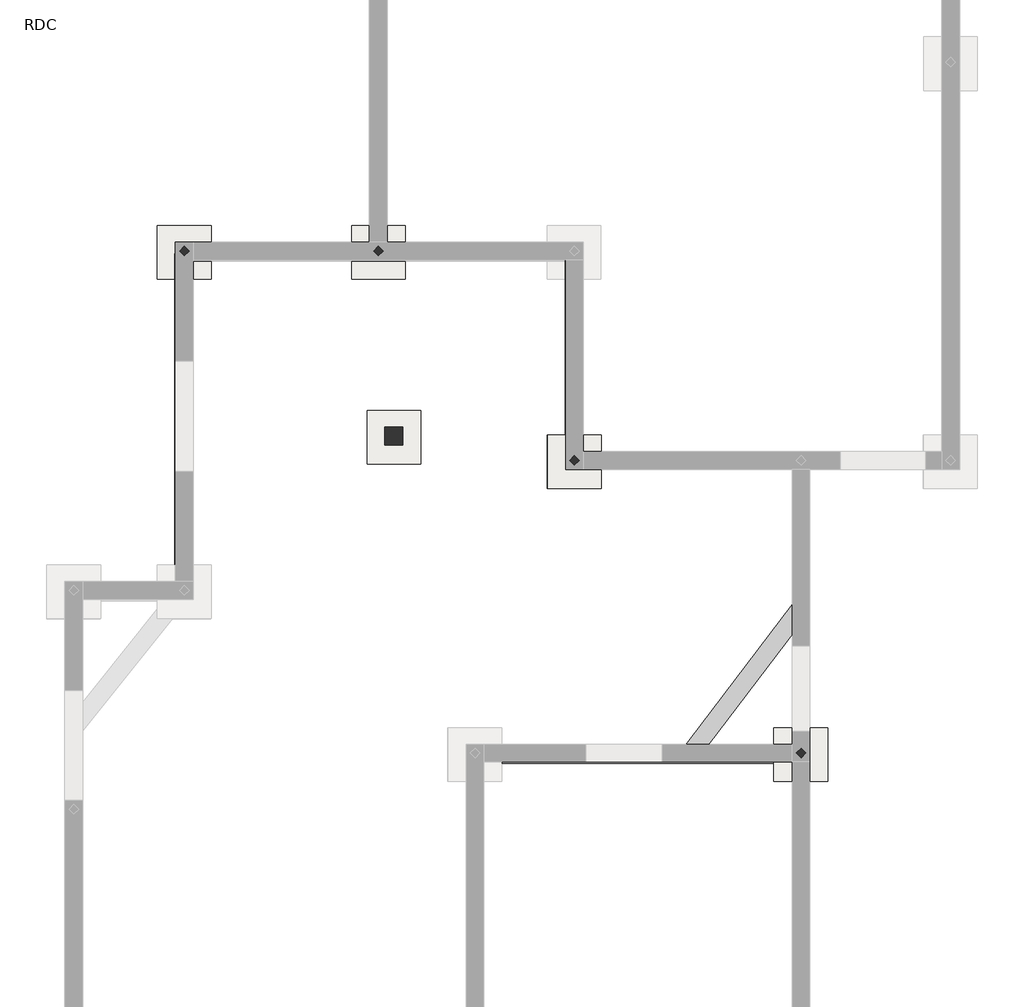
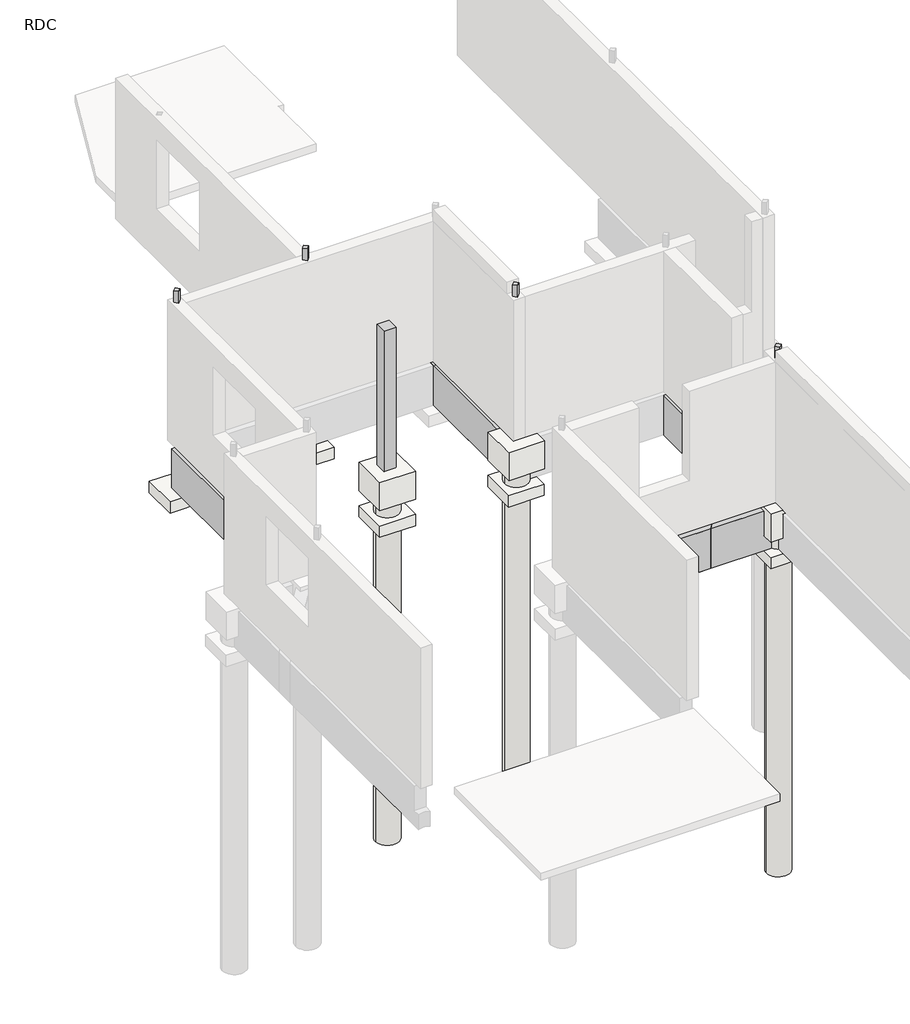
# One storey, part 4 of 5: 11 slabs, 7 beams, 5 columns.
"""IFC4 building model written with IfcOpenShell, lengths in millimetres."""

from ifc_helpers import new_model, si_unit, point, frame, frame_2d, origin, origin_with_axes, place, context, project, spatial, polyline, circle_curve, trimmed, segment, composite_curve, outline, extrude, faceted_brep, element, save
from ifc_brep_helpers import plane_surface, cylinder_surface, revolved_surface, advanced_brep

model = new_model("IFC4")

# Units and contexts
model_context = context("Model", 3, world=origin())
ifc_project = project(units=[si_unit("LENGTHUNIT", "METRE", prefix="MILLI")], contexts=[model_context])

# Site, building, storey
site = spatial("IfcSite", under=ifc_project)
building = spatial("IfcBuilding", under=site)
storey = spatial("IfcBuildingStorey", under=building, Name="RDC", Elevation=0.0)

# Beams
placement = place(None, origin())
element("IfcBeam", 1, ObjectType="Longrine BA : 20x70ht", at=placement, inside=storey, context=model_context, shape_type="AdvancedBrep", body=[
    advanced_brep(
    [(-4817.1649422, 2835.3224776, -67.0), (-4817.1649422, 2835.3224776, -767.0), (-4904.4649416, 2835.3224776, -767.0), (-5017.1649422, 2835.3224776, -767.0), (-5017.1649422, 2835.3224776, -67.0), (-4904.4649416, 2835.3224776, -67.0), (-4817.1649422, 2748.0224782, -67.0), (-4817.1649422, -644.3733983, -67.0), (-4817.1649422, -644.3733983, -500.0), (-4817.1649422, -768.6233971, -500.0), (-4817.1649422, -768.6233971, -767.0), (-4817.1649422, 2748.0224782, -767.0), (-5017.1649422, -773.8722262, -767.0), (-5017.1649422, -773.8722262, -500.0), (-5017.1649422, -644.3733983, -500.0), (-5017.1649422, -644.3733983, -67.0)],
    [
        (0, 1),
        (1, 2),
        (2, 3),
        (3, 4),
        (4, 5),
        (5, 0),
        (0, 6),
        (6, 7),
        (7, 8),
        (8, 9),
        (9, 10),
        (10, 11),
        (11, 1),
        (10, 12, circle_curve(frame((-4912.6214092, -944.3733983, -767.0), z_axis=(0.0, 0.0, 1.0), x_axis=(1.0, 0.0, 0.0)), 200.0)),
        (12, 3),
        (12, 13),
        (13, 14),
        (14, 15),
        (15, 4),
        (15, 7),
        (9, 13, circle_curve(frame((-4912.6214092, -944.3733983, -500.0), z_axis=(0.0, 0.0, 1.0), x_axis=(1.0, 0.0, 0.0)), 200.0)),
        (8, 14),
    ],
    [
        plane_surface(frame((-4817.1649422, 2835.3224776, -67.0), z_axis=(0.0, 1.0, 0.0), x_axis=(0.0, 0.0, -1.0))),
        plane_surface(frame((-4817.1649422, 2835.3224776, -67.0), z_axis=(1.0, 0.0, 0.0), x_axis=(0.0, -1.0, 0.0))),
        plane_surface(frame((-4817.1649422, 2835.3224776, -767.0), z_axis=(0.0, 0.0, -1.0), x_axis=(0.0, -1.0, 0.0))),
        plane_surface(frame((-5017.1649422, 2835.3224776, -767.0), z_axis=(-1.0, 0.0, 0.0), x_axis=(0.0, -1.0, 0.0))),
        plane_surface(frame((-5017.1649422, 2835.3224776, -67.0), z_axis=(0.0, 0.0, 1.0), x_axis=(0.0, -1.0, 0.0))),
        revolved_surface(polyline([(-4712.6214092, -944.3733983, -500.0), (-4712.6214092, -944.3733983, -767.0)]), (-4912.6214092, -944.3733983, -6600.0), (0.0, 0.0, 1.0)),
        plane_surface(frame((-5212.6214092, -644.3733983, -500.0), z_axis=(0.0, 0.0, 1.0), x_axis=(1.0, 0.0, 0.0))),
        plane_surface(frame((-4612.6214092, -644.3733983, 0.0), z_axis=(0.0, -1.0, 0.0), x_axis=(0.0, 0.0, -1.0))),
    ],
    [
        (0, [[1, 2, 3, 4, 5, 6]]),
        (1, [[-1, 7, 8, 9, 10, 11, 12, 13]]),
        (2, [[-3, -2, -13, -12, 14, 15]]),
        (3, [[-4, -15, 16, 17, 18, 19]]),
        (4, [[-6, -5, -19, 20, -8, -7]]),
        (5, [[-14, -11, 21, -16]]),
        (6, [[22, -17, -21, -10]]),
        (7, [[-22, -9, -20, -18]]),
    ],
),
])
element("IfcBeam", 2, ObjectType="Longrine BA : 20x70ht", at=placement, inside=storey, context=model_context, shape_type="AdvancedBrep", body=[
    advanced_brep(
    [(-659.9771125, 2835.3224776, -67.0), (-459.9771125, 2835.3224776, -67.0), (-459.9771125, 2835.3224776, -767.0), (-659.9771125, 2835.3224776, -767.0), (-659.9771125, 678.5236613, -767.0), (-659.9771125, 678.5236613, -500.0), (-659.9771125, 808.0224787, -500.0), (-659.9771125, 808.0224787, -67.0), (-459.9771125, 683.7724706, -767.0), (-459.9771125, 808.0224787, -67.0), (-459.9771125, 808.0224787, -500.0), (-459.9771125, 683.7724706, -500.0)],
    [
        (0, 1),
        (1, 2),
        (2, 3),
        (3, 0),
        (3, 4),
        (4, 5),
        (5, 6),
        (6, 7),
        (7, 0),
        (2, 8),
        (8, 4, circle_curve(frame((-555.4335965, 508.0224787, -767.0), z_axis=(0.0, 0.0, 1.0), x_axis=(1.0, 0.0, 0.0)), 200.0)),
        (1, 9),
        (9, 10),
        (10, 11),
        (11, 8),
        (7, 9),
        (11, 5, circle_curve(frame((-555.4335965, 508.0224787, -500.0), z_axis=(0.0, 0.0, 1.0), x_axis=(1.0, 0.0, 0.0)), 200.0)),
        (10, 6),
    ],
    [
        plane_surface(frame((-659.9771125, 2835.3224776, -67.0), z_axis=(0.0, 1.0, 0.0), x_axis=(0.0, 0.0, 1.0))),
        plane_surface(frame((-659.9771125, 536.535368, -417.0), z_axis=(-1.0, 0.0, 0.0), x_axis=(0.0, 0.0, -1.0))),
        plane_surface(frame((-559.9771125, 536.535368, -767.0), z_axis=(0.0, 0.0, -1.0), x_axis=(1.0, 0.0, 0.0))),
        plane_surface(frame((-459.9771125, 536.535368, -417.0), z_axis=(1.0, 0.0, 0.0), x_axis=(0.0, 0.0, 1.0))),
        plane_surface(frame((-559.9771125, 536.535368, -67.0), z_axis=(0.0, 0.0, 1.0), x_axis=(-1.0, 0.0, 0.0))),
        revolved_surface(polyline([(-355.4335965, 508.0224787, -500.0), (-355.4335965, 508.0224787, -767.0)]), (-555.4335965, 508.0224787, -6600.0), (0.0, 0.0, 1.0)),
        plane_surface(frame((-855.4335965, 808.0224787, -500.0), z_axis=(0.0, 0.0, 1.0), x_axis=(1.0, 0.0, 0.0))),
        plane_surface(frame((-255.4335965, 808.0224787, 0.0), z_axis=(0.0, -1.0, 0.0), x_axis=(0.0, 0.0, -1.0))),
    ],
    [
        (0, [[1, 2, 3, 4]]),
        (1, [[-4, 5, 6, 7, 8, 9]]),
        (2, [[-3, 10, 11, -5]]),
        (3, [[-2, 12, 13, 14, 15, -10]]),
        (4, [[-1, -9, 16, -12]]),
        (5, [[-11, -15, 17, -6]]),
        (6, [[18, -7, -17, -14]]),
        (7, [[-18, -13, -16, -8]]),
    ],
),
])
element("IfcBeam", 3, ObjectType="Longrine BA : 20x70ht", at=placement, inside=storey, context=model_context, shape_type="AdvancedBrep", body=[
    advanced_brep(
    [(1874.5663639, 423.8353673, -67.0), (1874.5663639, 423.8353673, -767.0), (1874.5663639, -2586.2275277, -767.0), (1874.5663639, -2586.2275277, -500.0), (1874.5663639, -2461.9775197, -500.0), (1874.5663639, -2461.9775197, -67.0), (2074.5663639, 423.8353673, -767.0), (2074.5663639, -2591.4763371, -767.0), (2074.5663639, 423.8353673, -67.0), (2074.5663639, -2461.9775197, -67.0), (2074.5663639, -2461.9775197, -500.0), (2074.5663639, -2591.4763371, -500.0)],
    [
        (0, 1),
        (1, 2),
        (2, 3),
        (3, 4),
        (4, 5),
        (5, 0),
        (1, 6),
        (6, 7),
        (7, 2, circle_curve(frame((1970.0228479, -2761.9775197, -767.0), z_axis=(0.0, 0.0, 1.0), x_axis=(1.0, 0.0, 0.0)), 200.0)),
        (6, 8),
        (8, 9),
        (9, 10),
        (10, 11),
        (11, 7),
        (8, 0),
        (5, 9),
        (11, 3, circle_curve(frame((1970.0228479, -2761.9775197, -500.0), z_axis=(0.0, 0.0, 1.0), x_axis=(1.0, 0.0, 0.0)), 200.0)),
        (10, 4),
    ],
    [
        plane_surface(frame((1874.5663639, -2749.277519, -417.0), z_axis=(-1.0, 0.0, 0.0), x_axis=(0.0, 0.0, -1.0))),
        plane_surface(frame((1974.5663639, -2749.277519, -767.0), z_axis=(0.0, 0.0, -1.0), x_axis=(1.0, 0.0, 0.0))),
        plane_surface(frame((2074.5663639, -2749.277519, -417.0), z_axis=(1.0, 0.0, 0.0), x_axis=(0.0, 0.0, 1.0))),
        plane_surface(frame((1974.5663639, -2749.277519, -67.0), z_axis=(0.0, 0.0, 1.0), x_axis=(-1.0, 0.0, 0.0))),
        revolved_surface(polyline([(2170.0228478999998, -2761.9775197, -500.0), (2170.0228478999998, -2761.9775197, -767.0)]), (1970.0228479, -2761.9775197, -6600.0), (0.0, 0.0, 1.0)),
        plane_surface(frame((3631.8663992, 423.8353673, -417.0), z_axis=(0.0, 1.0, 0.0), x_axis=(0.0, 0.0, -1.0))),
        plane_surface(frame((1670.0228479, -2461.9775197, -500.0), z_axis=(0.0, 0.0, 1.0), x_axis=(1.0, 0.0, 0.0))),
        plane_surface(frame((2270.0228479, -2461.9775197, 0.0), z_axis=(0.0, -1.0, 0.0), x_axis=(0.0, 0.0, -1.0))),
    ],
    [
        (0, [[1, 2, 3, 4, 5, 6]]),
        (1, [[7, 8, 9, -2]]),
        (2, [[10, 11, 12, 13, 14, -8]]),
        (3, [[15, -6, 16, -11]]),
        (4, [[-9, -14, 17, -3]]),
        (5, [[-1, -15, -10, -7]]),
        (6, [[18, -4, -17, -13]]),
        (7, [[-18, -12, -16, -5]]),
    ],
),
])
element("IfcBeam", 4, ObjectType="Longrine BA : 20x70ht", at=placement, inside=storey, context=model_context, shape_type="AdvancedBrep", body=[
    advanced_brep(
    [(1796.8177671, -2861.9775197, -767.0), (1796.8177671, -2861.9775197, -500.0), (1670.0228479, -2861.9775197, -500.0), (1670.0228479, -2861.9775197, -67.0), (-1366.4904447, -2861.9775197, -67.0), (-1366.4904447, -2861.9775197, -500.0), (-1491.844941, -2861.9775197, -500.0), (-1491.844941, -2861.9775197, -767.0), (-1466.4904447, -2764.5149728, -767.0), (-1494.7753589, -2661.9775197, -767.0), (1796.8177671, -2661.9775197, -767.0), (1770.0228479, -2761.9775197, -767.0), (1796.8177671, -2661.9775197, -500.0), (-1494.7753589, -2661.9775197, -500.0), (-1366.4904447, -2661.9775197, -500.0), (-1366.4904447, -2661.9775197, -67.0), (1670.0228479, -2661.9775197, -67.0), (1670.0228479, -2661.9775197, -500.0), (-1466.4904447, -2764.5149728, -500.0), (1770.0228479, -2761.9775197, -500.0)],
    [
        (0, 1),
        (1, 2),
        (2, 3),
        (3, 4),
        (4, 5),
        (5, 6),
        (6, 7),
        (7, 0),
        (7, 8, circle_curve(frame((-1666.4904447, -2764.5149728, -767.0), z_axis=(0.0, 0.0, 1.0), x_axis=(1.0, 0.0, 0.0)), 200.0)),
        (8, 9, circle_curve(frame((-1666.4904447, -2764.5149728, -767.0), z_axis=(0.0, 0.0, 1.0), x_axis=(1.0, 0.0, 0.0)), 200.0)),
        (9, 10),
        (10, 11, circle_curve(frame((1970.0228479, -2761.9775197, -767.0), z_axis=(0.0, 0.0, 1.0), x_axis=(1.0, 0.0, 0.0)), 200.0)),
        (11, 0, circle_curve(frame((1970.0228479, -2761.9775197, -767.0), z_axis=(0.0, 0.0, 1.0), x_axis=(1.0, 0.0, 0.0)), 200.0)),
        (12, 10),
        (9, 13),
        (13, 14),
        (14, 15),
        (15, 16),
        (16, 17),
        (17, 12),
        (3, 16),
        (15, 4),
        (6, 18, circle_curve(frame((-1666.4904447, -2764.5149728, -500.0), z_axis=(0.0, 0.0, 1.0), x_axis=(1.0, 0.0, 0.0)), 200.0)),
        (18, 8),
        (18, 13, circle_curve(frame((-1666.4904447, -2764.5149728, -500.0), z_axis=(0.0, 0.0, 1.0), x_axis=(1.0, 0.0, 0.0)), 200.0)),
        (11, 19),
        (19, 1, circle_curve(frame((1970.0228479, -2761.9775197, -500.0), z_axis=(0.0, 0.0, 1.0), x_axis=(1.0, 0.0, 0.0)), 200.0)),
        (12, 19, circle_curve(frame((1970.0228479, -2761.9775197, -500.0), z_axis=(0.0, 0.0, 1.0), x_axis=(1.0, 0.0, 0.0)), 200.0)),
        (17, 2),
        (5, 14),
    ],
    [
        plane_surface(frame((1961.8663633, -2861.9775197, -417.0), z_axis=(0.0, -1.0, 0.0), x_axis=(0.0, 0.0, -1.0))),
        plane_surface(frame((1961.8663633, -2761.9775197, -767.0), z_axis=(0.0, 0.0, -1.0), x_axis=(0.0, 1.0, 0.0))),
        plane_surface(frame((1961.8663633, -2661.9775197, -417.0), z_axis=(0.0, 1.0, 0.0), x_axis=(0.0, 0.0, 1.0))),
        plane_surface(frame((1961.8663633, -2761.9775197, -67.0), z_axis=(0.0, 0.0, 1.0), x_axis=(0.0, -1.0, 0.0))),
        revolved_surface(polyline([(-1466.4904447, -2764.5149728, -500.0), (-1466.4904447, -2764.5149728, -767.0)]), (-1666.4904447, -2764.5149728, -6600.0), (0.0, 0.0, 1.0)),
        revolved_surface(polyline([(2170.0228478999998, -2761.9775197, -500.0), (2170.0228478999998, -2761.9775197, -767.0)]), (1970.0228479, -2761.9775197, -6600.0), (0.0, 0.0, 1.0)),
        plane_surface(frame((1670.0228479, -2461.9775197, -500.0), z_axis=(0.0, 0.0, 1.0), x_axis=(1.0, 0.0, 0.0))),
        plane_surface(frame((1670.0228479, -2461.9775197, 0.0), z_axis=(1.0, 0.0, 0.0), x_axis=(0.0, 0.0, -1.0))),
        plane_surface(frame((-1966.4904447, -2464.5149728, -500.0), z_axis=(0.0, 0.0, 1.0), x_axis=(1.0, 0.0, 0.0))),
        plane_surface(frame((-1366.4904447, -3064.5149728, 0.0), z_axis=(-1.0, 0.0, 0.0), x_axis=(0.0, 0.0, -1.0))),
    ],
    [
        (0, [[1, 2, 3, 4, 5, 6, 7, 8]]),
        (1, [[9, 10, 11, 12, 13, -8]]),
        (2, [[14, -11, 15, 16, 17, 18, 19, 20]]),
        (3, [[21, -18, 22, -4]]),
        (4, [[-9, -7, 23, 24]]),
        (4, [[-10, -24, 25, -15]]),
        (5, [[-1, -13, 26, 27]]),
        (5, [[-26, -12, -14, 28]]),
        (6, [[29, -2, -27, -28, -20]]),
        (7, [[-29, -19, -21, -3]]),
        (8, [[30, -16, -25, -23, -6]]),
        (9, [[-30, -5, -22, -17]]),
    ],
),
])
element("IfcBeam", 5, ObjectType="Longrine BA : 20x70ht", at=placement, inside=storey, context=model_context, shape_type="SweptSolid", body=[
    extrude(outline(polyline([(2074.5663639, -830.5010844), (2074.5663639, -1160.7070139), (779.5785033, -2861.9775197), (528.2294858, -2861.9775197), (2074.5663639, -830.5010844)])), frame((0.0, 0.0, -767.0), z_axis=(0.0, 0.0, 1.0), x_axis=(1.0, 0.0, 0.0)), (0.0, 0.0, 1.0), 700.0),
])
element("IfcBeam", 6, ObjectType="Longrine BA : 20x70ht", at=placement, inside=storey, context=model_context, shape_type="AdvancedBrep", body=[
    advanced_brep(
    [(-459.9771125, 2835.3224776, -67.0), (-459.9771125, 2835.3224776, -767.0), (-572.6771131, 2835.3224776, -767.0), (-572.6771131, 2835.3224776, -67.0), (-459.9771125, 808.0224787, -67.0), (-459.9771125, 808.0224787, -500.0), (-459.9771125, 683.7724706, -500.0), (-459.9771125, 683.7724706, -767.0), (-659.9771125, 678.5236613, -767.0), (-659.9771125, 2748.0224782, -767.0), (-572.6771131, 2748.0224782, -767.0), (-659.9771125, 2748.0224782, -67.0), (-659.9771125, 678.5236613, -500.0), (-659.9771125, 808.0224787, -500.0), (-659.9771125, 808.0224787, -67.0), (-572.6771131, 2748.0224782, -67.0)],
    [
        (0, 1),
        (1, 2),
        (2, 3),
        (3, 0),
        (0, 4),
        (4, 5),
        (5, 6),
        (6, 7),
        (7, 1),
        (7, 8, circle_curve(frame((-555.4335965, 508.0224787, -767.0), z_axis=(0.0, 0.0, 1.0), x_axis=(1.0, 0.0, 0.0)), 200.0)),
        (8, 9),
        (9, 10),
        (10, 2),
        (11, 9),
        (8, 12),
        (12, 13),
        (13, 14),
        (14, 11),
        (3, 15),
        (15, 11),
        (14, 4),
        (15, 10),
        (6, 12, circle_curve(frame((-555.4335965, 508.0224787, -500.0), z_axis=(0.0, 0.0, 1.0), x_axis=(1.0, 0.0, 0.0)), 200.0)),
        (5, 13),
    ],
    [
        plane_surface(frame((-459.9771125, 2835.3224776, -67.0), z_axis=(0.0, 1.0, 0.0), x_axis=(0.0, 0.0, -1.0))),
        plane_surface(frame((-459.9771125, 2835.3224776, -417.0), z_axis=(1.0, 0.0, 0.0), x_axis=(0.0, 0.0, -1.0))),
        plane_surface(frame((-559.9771125, 2835.3224776, -767.0), z_axis=(0.0, 0.0, -1.0), x_axis=(-1.0, 0.0, 0.0))),
        plane_surface(frame((-659.9771125, 2835.3224776, -417.0), z_axis=(-1.0, 0.0, 0.0), x_axis=(0.0, 0.0, 1.0))),
        plane_surface(frame((-559.9771125, 2835.3224776, -67.0), z_axis=(0.0, 0.0, 1.0), x_axis=(1.0, 0.0, 0.0))),
        plane_surface(frame((-4904.4649416, 2748.0224782, -417.0), z_axis=(0.0, 1.0, 0.0), x_axis=(0.0, 0.0, 1.0))),
        revolved_surface(polyline([(-355.4335965, 508.0224787, -500.0), (-355.4335965, 508.0224787, -767.0)]), (-555.4335965, 508.0224787, -6600.0), (0.0, 0.0, 1.0)),
        plane_surface(frame((-572.6771131, 2948.0224782, -67.0), z_axis=(-1.0, 0.0, 0.0), x_axis=(0.0, 0.0, 1.0))),
        plane_surface(frame((-855.4335965, 808.0224787, -500.0), z_axis=(0.0, 0.0, 1.0), x_axis=(1.0, 0.0, 0.0))),
        plane_surface(frame((-255.4335965, 808.0224787, 0.0), z_axis=(0.0, -1.0, 0.0), x_axis=(0.0, 0.0, -1.0))),
    ],
    [
        (0, [[1, 2, 3, 4]]),
        (1, [[-1, 5, 6, 7, 8, 9]]),
        (2, [[-2, -9, 10, 11, 12, 13]]),
        (3, [[14, -11, 15, 16, 17, 18]]),
        (4, [[-4, 19, 20, -18, 21, -5]]),
        (5, [[22, -12, -14, -20]]),
        (6, [[-10, -8, 23, -15]]),
        (7, [[-22, -19, -3, -13]]),
        (8, [[24, -16, -23, -7]]),
        (9, [[-24, -6, -21, -17]]),
    ],
),
])
element("IfcBeam", 7, ObjectType="Longrine BA : 20x70ht", at=placement, inside=storey, context=model_context, shape_type="AdvancedBrep", body=[
    advanced_brep(
    [(678.0743146, -2861.9775197, -767.0), (1796.8177671, -2861.9775197, -767.0), (1796.8177671, -2861.9775197, -500.0), (1670.0228479, -2861.9775197, -500.0), (1670.0228479, -2861.9775197, -67.0), (678.0743146, -2861.9775197, -67.0), (678.0743146, -2665.1211664, -767.0), (680.4672229, -2661.9775197, -767.0), (1796.8177671, -2661.9775197, -767.0), (1770.0228479, -2761.9775197, -767.0), (680.4672229, -2661.9775197, -67.0), (1670.0228479, -2661.9775197, -67.0), (1670.0228479, -2661.9775197, -500.0), (1796.8177671, -2661.9775197, -500.0), (678.0743146, -2665.1211664, -67.0), (1770.0228479, -2761.9775197, -500.0)],
    [
        (0, 1),
        (1, 2),
        (2, 3),
        (3, 4),
        (4, 5),
        (5, 0),
        (0, 6),
        (6, 7),
        (7, 8),
        (8, 9, circle_curve(frame((1970.0228479, -2761.9775197, -767.0), z_axis=(0.0, 0.0, 1.0), x_axis=(1.0, 0.0, 0.0)), 200.0)),
        (9, 1, circle_curve(frame((1970.0228479, -2761.9775197, -767.0), z_axis=(0.0, 0.0, 1.0), x_axis=(1.0, 0.0, 0.0)), 200.0)),
        (7, 10),
        (10, 11),
        (11, 12),
        (12, 13),
        (13, 8),
        (14, 5),
        (4, 11),
        (10, 14),
        (9, 15),
        (15, 2, circle_curve(frame((1970.0228479, -2761.9775197, -500.0), z_axis=(0.0, 0.0, 1.0), x_axis=(1.0, 0.0, 0.0)), 200.0)),
        (13, 15, circle_curve(frame((1970.0228479, -2761.9775197, -500.0), z_axis=(0.0, 0.0, 1.0), x_axis=(1.0, 0.0, 0.0)), 200.0)),
        (12, 3),
        (14, 6),
    ],
    [
        plane_surface(frame((1961.8663633, -2861.9775197, -67.0), z_axis=(0.0, -1.0, 0.0), x_axis=(-1.0, 0.0, 0.0))),
        plane_surface(frame((1961.8663633, -2861.9775197, -767.0), z_axis=(0.0, 0.0, -1.0), x_axis=(-1.0, 0.0, 0.0))),
        plane_surface(frame((1961.8663633, -2661.9775197, -767.0), z_axis=(0.0, 1.0, 0.0), x_axis=(-1.0, 0.0, 0.0))),
        plane_surface(frame((1961.8663633, -2661.9775197, -67.0), z_axis=(0.0, 0.0, 1.0), x_axis=(-1.0, 0.0, 0.0))),
        revolved_surface(polyline([(2170.0228478999998, -2761.9775197, -500.0), (2170.0228478999998, -2761.9775197, -767.0)]), (1970.0228479, -2761.9775197, -6600.0), (0.0, 0.0, 1.0)),
        plane_surface(frame((1670.0228479, -2461.9775197, -500.0), z_axis=(0.0, 0.0, 1.0), x_axis=(1.0, 0.0, 0.0))),
        plane_surface(frame((1670.0228479, -2461.9775197, 0.0), z_axis=(1.0, 0.0, 0.0), x_axis=(0.0, 0.0, -1.0))),
        plane_surface(frame((678.0743146, -2761.9775197, -417.0), z_axis=(-1.0, 0.0, 0.0), x_axis=(0.0, -1.0, 0.0))),
        plane_surface(frame((571.6677663, -2804.9111426, -67.0), z_axis=(-0.7957063128923657, 0.605682642663001, 0.0), x_axis=(0.605682642663001, 0.7957063128923657, 0.0))),
    ],
    [
        (0, [[1, 2, 3, 4, 5, 6]]),
        (1, [[-1, 7, 8, 9, 10, 11]]),
        (2, [[12, 13, 14, 15, 16, -9]]),
        (3, [[17, -5, 18, -13, 19]]),
        (4, [[-11, 20, 21, -2]]),
        (4, [[-10, -16, 22, -20]]),
        (5, [[23, -3, -21, -22, -15]]),
        (6, [[-23, -14, -18, -4]]),
        (7, [[-6, -17, 24, -7]]),
        (8, [[-8, -24, -19, -12]]),
    ],
),
])

# Columns
element("IfcColumn", 8, ObjectType="CV : CV", at=placement, inside=storey, context=model_context, shape_type="Brep", body=[
    faceted_brep([(-4912.6214092, 2916.8683755, 2710.0), (-4965.6544178, 2863.8353669, 2710.0), (-4912.6214092, 2810.8023583, 2710.0), (-4859.5884006, 2863.8353669, 2710.0), (-4912.6214092, 2916.8683755, 0.0), (-4859.5884006, 2863.8353669, 0.0), (-4912.6214092, 2810.8023583, 0.0), (-4965.6544178, 2863.8353669, 0.0), (-4912.6214092, 2916.8683755, 2500.0), (-4965.6544178, 2863.8353669, 2500.0), (-4912.6214092, 2810.8023583, 2500.0), (-4859.5884006, 2863.8353669, 2500.0)], [[[0, 1, 2, 3]], [[4, 5, 6, 7]], [[1, 0, 8, 4, 7, 9]], [[2, 1, 9, 7, 6, 10]], [[3, 2, 10, 6, 5, 11]], [[0, 3, 11, 5, 4, 8]]]),
    faceted_brep([(-4859.5884006, 2863.8353669, 2710.0), (-4912.6214092, 2916.8683755, 2710.0), (-4965.6544178, 2863.8353669, 2710.0), (-4912.6214092, 2810.8023583, 2710.0), (-4859.5884006, 2863.8353669, 0.0), (-4912.6214092, 2810.8023583, 0.0), (-4965.6544178, 2863.8353669, 0.0), (-4912.6214092, 2916.8683755, 0.0), (-4859.5884006, 2863.8353669, 2500.0), (-4912.6214092, 2916.8683755, 2500.0), (-4965.6544178, 2863.8353669, 2500.0), (-4912.6214092, 2810.8023583, 2500.0)], [[[0, 1, 2, 3]], [[4, 5, 6, 7]], [[1, 0, 8, 4, 7, 9]], [[2, 1, 9, 7, 6, 10]], [[3, 2, 10, 6, 5, 11]], [[0, 3, 11, 5, 4, 8]]]),
])
element("IfcColumn", 9, ObjectType="CV : CV", at=placement, inside=storey, context=model_context, shape_type="Brep", body=[
    faceted_brep([(-2745.4336004, 2916.8683755, 2710.0), (-2798.466609, 2863.8353669, 2710.0), (-2745.4336004, 2810.8023583, 2710.0), (-2692.4005918, 2863.8353669, 2710.0), (-2745.4336004, 2916.8683755, 0.0), (-2692.4005918, 2863.8353669, 0.0), (-2745.4336004, 2810.8023583, 0.0), (-2798.466609, 2863.8353669, 0.0), (-2745.4336004, 2916.8683755, 2500.0), (-2798.466609, 2863.8353669, 2500.0), (-2745.4336004, 2810.8023583, 2500.0), (-2692.4005918, 2863.8353669, 2500.0)], [[[0, 1, 2, 3]], [[4, 5, 6, 7]], [[1, 0, 8, 4, 7, 9]], [[2, 1, 9, 7, 6, 10]], [[3, 2, 10, 6, 5, 11]], [[0, 3, 11, 5, 4, 8]]]),
    faceted_brep([(-2692.4005918, 2863.8353669, 2710.0), (-2745.4336004, 2916.8683755, 2710.0), (-2798.466609, 2863.8353669, 2710.0), (-2745.4336004, 2810.8023583, 2710.0), (-2692.4005918, 2863.8353669, 0.0), (-2745.4336004, 2810.8023583, 0.0), (-2798.466609, 2863.8353669, 0.0), (-2745.4336004, 2916.8683755, 0.0), (-2692.4005918, 2863.8353669, 2500.0), (-2745.4336004, 2916.8683755, 2500.0), (-2798.466609, 2863.8353669, 2500.0), (-2745.4336004, 2810.8023583, 2500.0)], [[[0, 1, 2, 3]], [[4, 5, 6, 7]], [[1, 0, 8, 4, 7, 9]], [[2, 1, 9, 7, 6, 10]], [[3, 2, 10, 6, 5, 11]], [[0, 3, 11, 5, 4, 8]]]),
])
element("IfcColumn", 10, ObjectType="CV : CV", at=placement, inside=storey, context=model_context, shape_type="Brep", body=[
    faceted_brep([(-555.4335965, 576.8683759, 2710.0), (-608.4666051, 523.8353673, 2710.0), (-555.4335965, 470.8023588, 2710.0), (-502.4005879, 523.8353673, 2710.0), (-555.4335965, 576.8683759, 0.0), (-502.4005879, 523.8353673, 0.0), (-555.4335965, 470.8023588, 0.0), (-608.4666051, 523.8353673, 0.0), (-555.4335965, 576.8683759, 2500.0), (-608.4666051, 523.8353673, 2500.0), (-555.4335965, 470.8023588, 2500.0), (-502.4005879, 523.8353673, 2500.0)], [[[0, 1, 2, 3]], [[4, 5, 6, 7]], [[1, 0, 8, 4, 7, 9]], [[2, 1, 9, 7, 6, 10]], [[3, 2, 10, 6, 5, 11]], [[0, 3, 11, 5, 4, 8]]]),
    faceted_brep([(-502.4005879, 523.8353673, 2710.0), (-555.4335965, 576.8683759, 2710.0), (-608.4666051, 523.8353673, 2710.0), (-555.4335965, 470.8023588, 2710.0), (-502.4005879, 523.8353673, 0.0), (-555.4335965, 470.8023588, 0.0), (-608.4666051, 523.8353673, 0.0), (-555.4335965, 576.8683759, 0.0), (-502.4005879, 523.8353673, 2500.0), (-555.4335965, 576.8683759, 2500.0), (-608.4666051, 523.8353673, 2500.0), (-555.4335965, 470.8023588, 2500.0)], [[[0, 1, 2, 3]], [[4, 5, 6, 7]], [[1, 0, 8, 4, 7, 9]], [[2, 1, 9, 7, 6, 10]], [[3, 2, 10, 6, 5, 11]], [[0, 3, 11, 5, 4, 8]]]),
])
element("IfcColumn", 11, ObjectType="CV : CV", at=placement, inside=storey, context=model_context, shape_type="Brep", body=[
    faceted_brep([(1974.5663639, -2693.1316224, 2710.0), (1921.5333553, -2746.164631, 2710.0), (1974.5663639, -2799.1976396, 2710.0), (2027.5993725, -2746.164631, 2710.0), (1974.5663639, -2693.1316224, 0.0), (2027.5993725, -2746.164631, 0.0), (1974.5663639, -2799.1976396, 0.0), (1921.5333553, -2746.164631, 0.0), (1974.5663639, -2693.1316224, 2500.0), (1921.5333553, -2746.164631, 2500.0), (1974.5663639, -2799.1976396, 2500.0), (2027.5993725, -2746.164631, 2500.0)], [[[0, 1, 2, 3]], [[4, 5, 6, 7]], [[1, 0, 8, 4, 7, 9]], [[2, 1, 9, 7, 6, 10]], [[3, 2, 10, 6, 5, 11]], [[0, 3, 11, 5, 4, 8]]]),
    faceted_brep([(2027.5993725, -2746.164631, 2710.0), (1974.5663639, -2693.1316224, 2710.0), (1921.5333553, -2746.164631, 2710.0), (1974.5663639, -2799.1976396, 2710.0), (2027.5993725, -2746.164631, 0.0), (1974.5663639, -2799.1976396, 0.0), (1921.5333553, -2746.164631, 0.0), (1974.5663639, -2693.1316224, 0.0), (2027.5993725, -2746.164631, 2500.0), (1974.5663639, -2693.1316224, 2500.0), (1921.5333553, -2746.164631, 2500.0), (1974.5663639, -2799.1976396, 2500.0)], [[[0, 1, 2, 3]], [[4, 5, 6, 7]], [[1, 0, 8, 4, 7, 9]], [[2, 1, 9, 7, 6, 10]], [[3, 2, 10, 6, 5, 11]], [[0, 3, 11, 5, 4, 8]]]),
])
element("IfcColumn", 12, ObjectType="Poteau BA : 20x20", at=placement, inside=storey, context=model_context, shape_type="SweptSolid", body=[
    extrude(outline(polyline([(-2475.4327864, 897.5075352), (-2475.4327864, 697.5075352), (-2675.4327864, 697.5075352), (-2675.4327864, 897.5075352), (-2475.4327864, 897.5075352)])), origin_with_axes(), (0.0, 0.0, 1.0), 2500.0),
])

# Slabs
element("IfcSlab", 13, ObjectType="Pieu-Conduite en acier : Diamètre de 400 mm", at=placement, inside=storey, context=model_context, shape_type="SweptSolid", body=[
    extrude(outline(composite_curve([segment(trimmed(circle_curve(frame_2d((-2571.8171747, 781.6946465)), 200.0), [point((-2771.8171747, 781.6946465))], [point((-2371.8171747, 781.6946465))], False, "CARTESIAN"), True, "CONTINUOUS"), segment(trimmed(circle_curve(frame_2d((-2571.8171747, 781.6946465)), 200.0), [point((-2371.8171747, 781.6946465))], [point((-2771.8171747, 781.6946465))], False, "CARTESIAN"), True, "CONTINUOUS")], self_intersect=False)), frame((0.0, 0.0, -6600.0), z_axis=(0.0, 0.0, 1.0), x_axis=(1.0, 0.0, 0.0)), (0.0, 0.0, 1.0), 5630.0),
    extrude(outline(composite_curve([segment(trimmed(circle_curve(frame_2d((-2571.8171747, 781.6946465)), 200.0), [point((-2371.8171747, 781.6946465))], [point((-2771.8171747, 781.6946465))], False, "CARTESIAN"), True, "CONTINUOUS"), segment(trimmed(circle_curve(frame_2d((-2571.8171747, 781.6946465)), 200.0), [point((-2771.8171747, 781.6946465))], [point((-2371.8171747, 781.6946465))], False, "CARTESIAN"), True, "CONTINUOUS")], self_intersect=False)), frame((0.0, 0.0, -770.0), z_axis=(0.0, 0.0, 1.0), x_axis=(1.0, 0.0, 0.0)), (0.0, 0.0, 1.0), 270.0),
])
element("IfcSlab", 14, ObjectType="Pieu-Conduite en acier : Diamètre de 400 mm", at=placement, inside=storey, context=model_context, shape_type="AdvancedBrep", body=[
    advanced_brep(
    [(-755.4335965, 508.0224787, -6600.0), (-355.4335965, 508.0224787, -6600.0), (-755.4335965, 508.0224787, -970.0), (-355.4335965, 508.0224787, -970.0)],
    [
        (0, 1, circle_curve(frame((-555.4335965, 508.0224787, -6600.0), z_axis=(0.0, 0.0, -1.0), x_axis=(1.0, 0.0, 0.0)), 200.0)),
        (1, 0, circle_curve(frame((-555.4335965, 508.0224787, -6600.0), z_axis=(0.0, 0.0, -1.0), x_axis=(1.0, 0.0, 0.0)), 200.0)),
        (2, 3, circle_curve(frame((-555.4335965, 508.0224787, -970.0), z_axis=(0.0, 0.0, 1.0), x_axis=(1.0, 0.0, 0.0)), 200.0)),
        (3, 2, circle_curve(frame((-555.4335965, 508.0224787, -970.0), z_axis=(0.0, 0.0, 1.0), x_axis=(1.0, 0.0, 0.0)), 200.0)),
        (1, 3),
        (2, 0),
    ],
    [
        plane_surface(frame((-355.4335965, 508.0224787, -6600.0), z_axis=(0.0, 0.0, -1.0), x_axis=(0.0, -1.0, 0.0))),
        plane_surface(frame((-859.9771445, 808.0224787, -970.0), z_axis=(0.0, 0.0, 1.0), x_axis=(1.0, 0.0, 0.0))),
        cylinder_surface(frame((-555.4335965, 508.0224787, -6600.0), z_axis=(0.0, 0.0, 1.0), x_axis=(1.0, 0.0, 0.0)), 200.0),
    ],
    [
        (0, [[1, 2]]),
        (1, [[3, 4]]),
        (2, [[-2, 5, -3, 6]]),
        (2, [[-1, -6, -4, -5]]),
    ],
),
    advanced_brep(
    [(-755.4335965, 508.0224787, -770.0), (-355.4335965, 508.0224787, -770.0), (-355.4335965, 508.0224787, -500.0), (-374.0154875, 423.8353673, -500.0), (-755.4335965, 508.0224787, -500.0), (-659.9771125, 678.5236613, -500.0), (-459.9771125, 683.7724706, -500.0), (-392.3878332, 623.850278, -500.0)],
    [
        (0, 1, circle_curve(frame((-555.4335965, 508.0224787, -770.0), z_axis=(0.0, 0.0, 1.0), x_axis=(1.0, 0.0, 0.0)), 200.0)),
        (1, 2),
        (2, 3, circle_curve(frame((-555.4335965, 508.0224787, -500.0), z_axis=(0.0, 0.0, -1.0), x_axis=(1.0, 0.0, 0.0)), 200.0)),
        (3, 4, circle_curve(frame((-555.4335965, 508.0224787, -500.0), z_axis=(0.0, 0.0, -1.0), x_axis=(1.0, 0.0, 0.0)), 200.0)),
        (4, 0),
        (1, 0, circle_curve(frame((-555.4335965, 508.0224787, -770.0), z_axis=(0.0, 0.0, 1.0), x_axis=(1.0, 0.0, 0.0)), 200.0)),
        (4, 5, circle_curve(frame((-555.4335965, 508.0224787, -500.0), z_axis=(0.0, 0.0, -1.0), x_axis=(1.0, 0.0, 0.0)), 200.0)),
        (5, 6, circle_curve(frame((-555.4335965, 508.0224787, -500.0), z_axis=(0.0, 0.0, -1.0), x_axis=(1.0, 0.0, 0.0)), 200.0)),
        (6, 7, circle_curve(frame((-555.4335965, 508.0224787, -500.0), z_axis=(0.0, 0.0, -1.0), x_axis=(1.0, 0.0, 0.0)), 200.0)),
        (7, 2, circle_curve(frame((-555.4335965, 508.0224787, -500.0), z_axis=(0.0, 0.0, -1.0), x_axis=(1.0, 0.0, 0.0)), 200.0)),
    ],
    [
        cylinder_surface(frame((-555.4335965, 508.0224787, -6600.0), z_axis=(0.0, 0.0, 1.0), x_axis=(1.0, 0.0, 0.0)), 200.0),
        plane_surface(frame((-859.9771445, 808.0224787, -770.0), z_axis=(0.0, 0.0, -1.0), x_axis=(-1.0, 0.0, 0.0))),
        plane_surface(frame((-855.4335965, 808.0224787, -500.0), z_axis=(0.0, 0.0, 1.0), x_axis=(1.0, 0.0, 0.0))),
    ],
    [
        (0, [[1, 2, 3, 4, 5]]),
        (0, [[6, -5, 7, 8, 9, 10, -2]]),
        (1, [[-1, -6]]),
        (2, [[-4, -3, -10, -9, -8, -7]]),
    ],
),
])
element("IfcSlab", 15, ObjectType="Pieu-Conduite en acier : Diamètre de 400 mm", at=placement, inside=storey, context=model_context, shape_type="AdvancedBrep", body=[
    advanced_brep(
    [(1770.0228479, -2761.9775197, -6600.0), (2170.0228479, -2761.9775197, -6600.0), (1770.0228479, -2761.9775197, -970.0), (2170.0228479, -2761.9775197, -970.0)],
    [
        (0, 1, circle_curve(frame((1970.0228479, -2761.9775197, -6600.0), z_axis=(0.0, 0.0, -1.0), x_axis=(1.0, 0.0, 0.0)), 200.0)),
        (1, 0, circle_curve(frame((1970.0228479, -2761.9775197, -6600.0), z_axis=(0.0, 0.0, -1.0), x_axis=(1.0, 0.0, 0.0)), 200.0)),
        (2, 3, circle_curve(frame((1970.0228479, -2761.9775197, -970.0), z_axis=(0.0, 0.0, 1.0), x_axis=(1.0, 0.0, 0.0)), 200.0)),
        (3, 2, circle_curve(frame((1970.0228479, -2761.9775197, -970.0), z_axis=(0.0, 0.0, 1.0), x_axis=(1.0, 0.0, 0.0)), 200.0)),
        (1, 3),
        (2, 0),
    ],
    [
        plane_surface(frame((2170.0228479, -2761.9775197, -6600.0), z_axis=(0.0, 0.0, -1.0), x_axis=(0.0, -1.0, 0.0))),
        plane_surface(frame((1670.0228479, -2461.9775197, -970.0), z_axis=(0.0, 0.0, 1.0), x_axis=(1.0, 0.0, 0.0))),
        cylinder_surface(frame((1970.0228479, -2761.9775197, -6600.0), z_axis=(0.0, 0.0, 1.0), x_axis=(1.0, 0.0, 0.0)), 200.0),
    ],
    [
        (0, [[1, 2]]),
        (1, [[3, 4]]),
        (2, [[-2, 5, -3, 6]]),
        (2, [[-1, -6, -4, -5]]),
    ],
),
    advanced_brep(
    [(1770.0228479, -2761.9775197, -770.0), (2170.0228479, -2761.9775197, -770.0), (2170.0228479, -2761.9775197, -500.0), (2074.5557716, -2932.4851965, -500.0), (1874.5489367, -2937.7180451, -500.0), (1796.8177671, -2861.9775197, -500.0), (1770.0228479, -2761.9775197, -500.0), (1796.8281566, -2661.9595268, -500.0), (1874.5663639, -2586.2275277, -500.0), (2074.5663639, -2591.4763371, -500.0)],
    [
        (0, 1, circle_curve(frame((1970.0228479, -2761.9775197, -770.0), z_axis=(0.0, 0.0, 1.0), x_axis=(1.0, 0.0, 0.0)), 200.0)),
        (1, 2),
        (2, 3, circle_curve(frame((1970.0228479, -2761.9775197, -500.0), z_axis=(0.0, 0.0, -1.0), x_axis=(1.0, 0.0, 0.0)), 200.0)),
        (3, 4, circle_curve(frame((1970.0228479, -2761.9775197, -500.0), z_axis=(0.0, 0.0, -1.0), x_axis=(1.0, 0.0, 0.0)), 200.0)),
        (4, 5, circle_curve(frame((1970.0228479, -2761.9775197, -500.0), z_axis=(0.0, 0.0, -1.0), x_axis=(1.0, 0.0, 0.0)), 200.0)),
        (5, 6, circle_curve(frame((1970.0228479, -2761.9775197, -500.0), z_axis=(0.0, 0.0, -1.0), x_axis=(1.0, 0.0, 0.0)), 200.0)),
        (6, 0),
        (1, 0, circle_curve(frame((1970.0228479, -2761.9775197, -770.0), z_axis=(0.0, 0.0, 1.0), x_axis=(1.0, 0.0, 0.0)), 200.0)),
        (6, 7, circle_curve(frame((1970.0228479, -2761.9775197, -500.0), z_axis=(0.0, 0.0, -1.0), x_axis=(1.0, 0.0, 0.0)), 200.0)),
        (7, 8, circle_curve(frame((1970.0228479, -2761.9775197, -500.0), z_axis=(0.0, 0.0, -1.0), x_axis=(1.0, 0.0, 0.0)), 200.0)),
        (8, 9, circle_curve(frame((1970.0228479, -2761.9775197, -500.0), z_axis=(0.0, 0.0, -1.0), x_axis=(1.0, 0.0, 0.0)), 200.0)),
        (9, 2, circle_curve(frame((1970.0228479, -2761.9775197, -500.0), z_axis=(0.0, 0.0, -1.0), x_axis=(1.0, 0.0, 0.0)), 200.0)),
    ],
    [
        cylinder_surface(frame((1970.0228479, -2761.9775197, -6600.0), z_axis=(0.0, 0.0, 1.0), x_axis=(1.0, 0.0, 0.0)), 200.0),
        plane_surface(frame((1670.0228479, -2461.9775197, -770.0), z_axis=(0.0, 0.0, -1.0), x_axis=(-1.0, 0.0, 0.0))),
        plane_surface(frame((1670.0228479, -2461.9775197, -500.0), z_axis=(0.0, 0.0, 1.0), x_axis=(1.0, 0.0, 0.0))),
    ],
    [
        (0, [[1, 2, 3, 4, 5, 6, 7]]),
        (0, [[8, -7, 9, 10, 11, 12, -2]]),
        (1, [[-1, -8]]),
        (2, [[-6, -5, -4, -3, -12, -11, -10, -9]]),
    ],
),
])
element("IfcSlab", 16, ObjectType="Tête de pieux-1 poteau : 60x60x50", at=placement, inside=storey, context=model_context, shape_type="SweptSolid", body=[
    extrude(outline(polyline([(-2271.8171747, 1081.6946465), (-2271.8171747, 481.6946465), (-2871.8171747, 481.6946465), (-2871.8171747, 1081.6946465), (-2271.8171747, 1081.6946465)])), frame((0.0, 0.0, -500.0), z_axis=(0.0, 0.0, 1.0), x_axis=(1.0, 0.0, 0.0)), (0.0, 0.0, 1.0), 500.0),
])
element("IfcSlab", 17, ObjectType="Tête de pieux-1 poteau : 60x60x50", at=placement, inside=storey, context=model_context, shape_type="Brep", body=[
    faceted_brep([(-255.4335965, 808.0224787, 0.0), (-855.4335965, 808.0224787, 0.0), (-855.4335965, 208.0224787, 0.0), (-255.4335965, 208.0224787, 0.0), (-255.4335965, 808.0224787, -500.0), (-255.4335965, 623.8353673, -500.0), (-255.4335965, 423.8353673, -500.0), (-255.4335965, 208.0224787, -500.0), (-855.4335965, 208.0224787, -500.0), (-855.4335965, 808.0224787, -500.0), (-659.9771125, 808.0224787, -500.0), (-459.9771125, 808.0224787, -500.0)], [[[0, 1, 2, 3]], [[4, 5, 6, 7, 8, 9, 10, 11]], [[1, 0, 4, 11, 10, 9]], [[2, 1, 9, 8]], [[3, 2, 8, 7]], [[0, 3, 7, 6, 5, 4]]]),
])
element("IfcSlab", 18, ObjectType="Tête de pieux-1 poteau : 60x60x50", at=placement, inside=storey, context=model_context, shape_type="Brep", body=[
    faceted_brep([(2270.0228479, -2461.9775197, 0.0), (1670.0228479, -2461.9775197, 0.0), (1670.0228479, -3061.9775197, 0.0), (2270.0228479, -3061.9775197, 0.0), (2270.0228479, -2461.9775197, -500.0), (2270.0228479, -3061.9775197, -500.0), (2074.5663639, -3061.9775197, -500.0), (1874.5663639, -3061.9775197, -500.0), (1670.0228479, -3061.9775197, -500.0), (1670.0228479, -2861.9775197, -500.0), (1670.0228479, -2661.9775197, -500.0), (1670.0228479, -2461.9775197, -500.0), (1874.5663639, -2461.9775197, -500.0), (2074.5663639, -2461.9775197, -500.0)], [[[0, 1, 2, 3]], [[4, 5, 6, 7, 8, 9, 10, 11, 12, 13]], [[1, 0, 4, 13, 12, 11]], [[2, 1, 11, 10, 9, 8]], [[3, 2, 8, 7, 6, 5]], [[0, 3, 5, 4]]]),
])
element("IfcSlab", 19, ObjectType="M_Base-Rectangulaire : 60x60x20", at=placement, inside=storey, context=model_context, shape_type="SweptSolid", body=[
    extrude(outline(polyline([(2270.0228479, -2461.9775197), (2270.0228479, -3061.9775197), (1670.0228479, -3061.9775197), (1670.0228479, -2461.9775197), (2270.0228479, -2461.9775197)])), frame((0.0, 0.0, -970.0), z_axis=(0.0, 0.0, 1.0), x_axis=(1.0, 0.0, 0.0)), (0.0, 0.0, 1.0), 200.0),
    extrude(outline(polyline([(2270.0228479, -2461.9775197), (2270.0228479, -3061.9775197), (1670.0228479, -3061.9775197), (1670.0228479, -2461.9775197), (2270.0228479, -2461.9775197)])), frame((0.0, 0.0, -970.0), z_axis=(0.0, 0.0, 1.0), x_axis=(1.0, 0.0, 0.0)), (0.0, 0.0, 1.0), 200.0),
])
element("IfcSlab", 20, ObjectType="M_Base-Rectangulaire : 60x60x20", at=placement, inside=storey, context=model_context, shape_type="SweptSolid", body=[
    extrude(outline(polyline([(-259.9771445, 808.0224787), (-259.9771445, 208.0224787), (-859.9771445, 208.0224787), (-859.9771445, 808.0224787), (-259.9771445, 808.0224787)])), frame((0.0, 0.0, -970.0), z_axis=(0.0, 0.0, 1.0), x_axis=(1.0, 0.0, 0.0)), (0.0, 0.0, 1.0), 200.0),
    extrude(outline(polyline([(-259.9771445, 808.0224787), (-259.9771445, 208.0224787), (-859.9771445, 208.0224787), (-859.9771445, 808.0224787), (-259.9771445, 808.0224787)])), frame((0.0, 0.0, -970.0), z_axis=(0.0, 0.0, 1.0), x_axis=(1.0, 0.0, 0.0)), (0.0, 0.0, 1.0), 200.0),
])
element("IfcSlab", 21, ObjectType="M_Base-Rectangulaire : 60x60x20", at=placement, inside=storey, context=model_context, shape_type="SweptSolid", body=[
    extrude(outline(polyline([(-2271.8171747, 1081.6946465), (-2271.8171747, 481.6946465), (-2871.8171747, 481.6946465), (-2871.8171747, 1081.6946465), (-2271.8171747, 1081.6946465)])), frame((0.0, 0.0, -970.0), z_axis=(0.0, 0.0, 1.0), x_axis=(1.0, 0.0, 0.0)), (0.0, 0.0, 1.0), 200.0),
    extrude(outline(polyline([(-2271.8171747, 1081.6946465), (-2271.8171747, 481.6946465), (-2871.8171747, 481.6946465), (-2871.8171747, 1081.6946465), (-2271.8171747, 1081.6946465)])), frame((0.0, 0.0, -970.0), z_axis=(0.0, 0.0, 1.0), x_axis=(1.0, 0.0, 0.0)), (0.0, 0.0, 1.0), 200.0),
])
element("IfcSlab", 22, ObjectType="M_Base-Rectangulaire : 60x60x20", at=placement, inside=storey, context=model_context, shape_type="Brep", body=[
    faceted_brep([(-2445.4336004, 3148.0224782, -770.0), (-2449.9542111, 3148.0224782, -770.0), (-3045.4336004, 3148.0224782, -770.0), (-3045.4336004, 2947.3616236, -770.0), (-3045.4336004, 2548.0224782, -770.0), (-2445.4336004, 2548.0224782, -770.0), (-2445.4336004, 3148.0224782, -970.0), (-2445.4336004, 2548.0224782, -970.0), (-3045.4336004, 2548.0224782, -970.0), (-3045.4336004, 2947.3616236, -970.0), (-3045.4336004, 3148.0224782, -970.0), (-2449.9542111, 3148.0224782, -970.0)], [[[0, 1, 2, 3, 4, 5]], [[6, 7, 8, 9, 10, 11]], [[2, 1, 0, 6, 11, 10]], [[4, 3, 2, 10, 9, 8]], [[5, 4, 8, 7]], [[0, 5, 7, 6]]]),
    faceted_brep([(-2445.4336004, 3148.0224782, -770.0), (-2449.9542111, 3148.0224782, -770.0), (-3045.4336004, 3148.0224782, -770.0), (-3045.4336004, 2947.3616236, -770.0), (-3045.4336004, 2548.0224782, -770.0), (-2445.4336004, 2548.0224782, -770.0), (-2445.4336004, 3148.0224782, -970.0), (-2445.4336004, 2548.0224782, -970.0), (-3045.4336004, 2548.0224782, -970.0), (-3045.4336004, 2947.3616236, -970.0), (-3045.4336004, 3148.0224782, -970.0), (-2449.9542111, 3148.0224782, -970.0)], [[[0, 1, 2, 3, 4, 5]], [[6, 7, 8, 9, 10, 11]], [[2, 1, 0, 6, 11, 10]], [[4, 3, 2, 10, 9, 8]], [[5, 4, 8, 7]], [[0, 5, 7, 6]]]),
])
element("IfcSlab", 23, ObjectType="M_Base-Rectangulaire : 60x60x20", at=placement, inside=storey, context=model_context, shape_type="SweptSolid", body=[
    extrude(outline(polyline([(-4612.6214092, 3148.0224782), (-4612.6214092, 2548.0224782), (-5212.6214092, 2548.0224782), (-5212.6214092, 3148.0224782), (-4612.6214092, 3148.0224782)])), frame((0.0, 0.0, -970.0), z_axis=(0.0, 0.0, 1.0), x_axis=(1.0, 0.0, 0.0)), (0.0, 0.0, 1.0), 200.0),
    extrude(outline(polyline([(-4612.6214092, 3148.0224782), (-4612.6214092, 2548.0224782), (-5212.6214092, 2548.0224782), (-5212.6214092, 3148.0224782), (-4612.6214092, 3148.0224782)])), frame((0.0, 0.0, -970.0), z_axis=(0.0, 0.0, 1.0), x_axis=(1.0, 0.0, 0.0)), (0.0, 0.0, 1.0), 200.0),
])

save(model, "model.ifc")

# Revit data of these elements
# Type "Longrine BA : 20x70ht"
#   Length [instance default] = 1.524 m
#   b = 0.200 m
#   h = 0.700 m
#   Structural Material = Maçonnerie - Béton
#   Assembly Code = ""
# Type "CV : CV"
#   Structural Material [instance default] = Béton coulé sur place
#   Default Elevation = 0
# Type "Poteau BA : 20x20"
#   b = 0.200 m
#   h = 0.200 m
#   Structural Material [instance default] = none
# Type "Pieu-Conduite en acier : Diamètre de 400 mm"
#   Assembly Code = "A1020130"
#   Rayon = 0.200 m
#   Enrobage minimum = 0.150 m
#   Diameter = 0.400 m
#   Depth = 6.000 m
#   Structural Material [instance default] = Métal - Acier - 345 MPa
# Type "Tête de pieux-1 poteau : 60x60x50"
#   Assembly Code = "A1010130"
#   Width = 0.600 m
#   Length = 0.600 m
#   Foundation Thickness = 0.500 m
#   Coupure = 0.050 m
#   Structural Material [instance default] = Béton - Béton coulé sur place
#   Type de pieu = Pieu-Conduite en acier : Diamètre de 400 mm
# Type "M_Base-Rectangulaire : 60x60x20"
#   Length = 0.600 m
#   Width = 0.600 m
#   Foundation Thickness = 0.200 m
#   Structural Material [instance default] = Béton - Béton coulé sur place
#   Assembly Code = ""
# Elements 1, 2, 3, 4, 5, 6, 7 (IfcBeam, "Longrine BA : 20x70ht")
#   Phase Created = Nouvelle construction
#   Materials on its faces: "Maçonnerie - Béton"
# Elements 8, 9, 10, 11 (IfcColumn, "CV : CV")
#   Structural Material = Béton coulé sur place
#   Phase Created = Nouvelle construction
#   Materials on its faces: "Béton coulé sur place"
# Element 12 (IfcColumn, "Poteau BA : 20x20")
#   Structural Material = Béton - Coulé sur place - Béton25
#   Phase Created = Nouvelle construction
#   Materials on its faces: "Béton - Coulé sur place - Béton25"
# Elements 13, 14, 15 (IfcSlab, "Pieu-Conduite en acier : Diamètre de 400 mm")
#   Structural Material = none
#   Phase Created = Nouvelle construction
# Elements 16, 17, 18 (IfcSlab, "Tête de pieux-1 poteau : 60x60x50")
#   Structural Material = Béton - Béton coulé sur place
#   Phase Created = Nouvelle construction
#   Materials on its faces: "Béton - Béton coulé sur place"
# Elements 19, 20, 21, 22, 23 (IfcSlab, "M_Base-Rectangulaire : 60x60x20")
#   Structural Material = Béton - Béton coulé sur place
#   Phase Created = Nouvelle construction
#   Materials on its faces: "Béton - Béton coulé sur place"
# Materials
#   "Maçonnerie - Béton": class "Béton", colour RGB 153 162 160, transparency 0, Cost = 0
#   "Béton coulé sur place": class "Béton", colour RGB 0 0 0, transparency 0, Description = "Matériau physique.", Cost = 0
#   "Métal - Acier - 345 MPa": class "Métal", colour RGB 247 247 247, transparency 0, Cost = 0
#   "Béton - Béton coulé sur place": class "Béton", colour RGB 192 192 192, transparency 0, Cost = 0
#   "Béton - Coulé sur place - Béton25": class "Béton", colour RGB 192 192 192, transparency 0, Cost = 0
